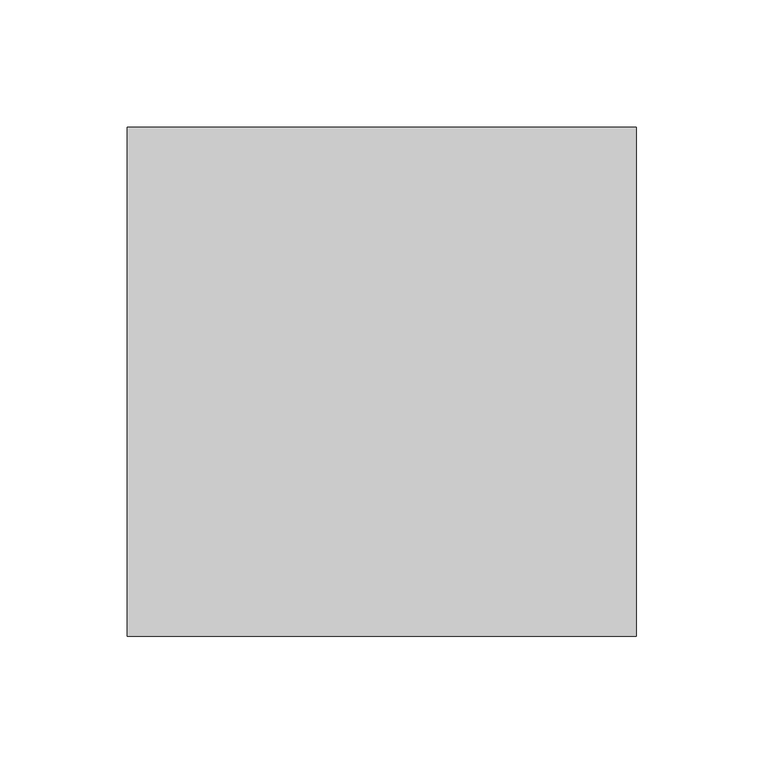
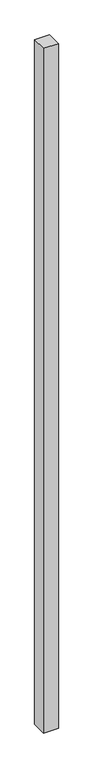
"""IFC4 building model written with IfcOpenShell, lengths in millimetres: proxy geometry, STptze."""

from ifc_helpers import new_model, si_unit, origin, origin_with_axes, place, context, project, spatial, polyline, outline, extrude, source, transform, mapped, element, save


def generic_models_f2156eff(model_context):
    return source(origin(), model_context, "Body", "SweptSolid", [
        extrude(outline(polyline([(163697.7593015, 40484.7962965), (163897.7593015, 40484.7962965), (163897.7593015, 40284.7962965), (163697.7593015, 40284.7962965), (163697.7593015, 40484.7962965)])), origin_with_axes(), (0.0, 0.0, 1.0), 9650.0),
    ])


if __name__ == "__main__":
    model = new_model("IFC4")
    model_context = context("Model", 3, world=origin())
    ifc_project = project(units=[si_unit("LENGTHUNIT", "METRE", prefix="MILLI")], contexts=[model_context])
    site = spatial("IfcSite", under=ifc_project)
    building = spatial("IfcBuilding", under=site)
    placement = place(None, origin())
    generic_models_shape = generic_models_f2156eff(model_context)
    element("IfcBuildingElementProxy", 1, Name="STptze", ObjectType="STptze", at=placement, inside=building, context=model_context, shape_type="MappedRepresentation", body=[
        mapped(generic_models_shape, transform((0.0, 0.0, 0.0), x_axis=(1.0, 0.0, 0.0), y_axis=(0.0, 1.0, 0.0), z_axis=(0.0, 0.0, 1.0))),
    ])
    save(model, "model.ifc")

# Revit data of these elements
# Element 1 (IfcBuildingElementProxy, "STptze")
#   Materials on its faces: "material wardrobe b 1"
# Materials
#   "material wardrobe b 1": class "Unassigned", colour RGB 128 128 128, transparency 0
